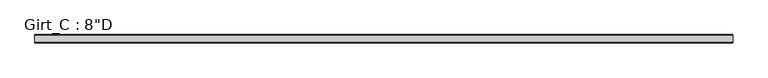
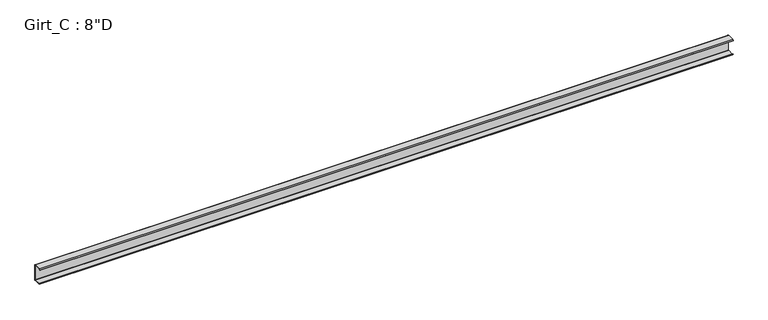
"""IFC4 building model written with IfcOpenShell, lengths in millimetres: beam geometry."""

import ifcopenshell
import ifcopenshell.guid

model = None  # the IFC model being written
_history = None  # IfcOwnerHistory: only IFC2X3 demands one
_inside = {}  # id of a spatial element -> (the spatial element, [elements in it])
_under = {}  # id of a project, library or spatial element -> (it, [spatial elements below it])
_declared = {}  # id of a project -> (the project, [libraries it declares])
_typed = {}  # id of a type object -> (the type object, [elements of that type])
_made_of = {}  # id of a material, layer set ... -> (it, [elements and type objects made of it])


def new_model(schema):
    """Start an empty IFC model of exactly this schema.

    Asked for "IFC4X3", IfcOpenShell would pick the latest addendum, in which some entities
    have other attributes; the version numbers below select the first issue.
    IFC2X3 requires an IfcOwnerHistory on every rooted entity: one is made here for all.
    """
    global model, _history
    if schema == "IFC4X3":
        model = ifcopenshell.file(schema_version=(4, 3, 0, 0))
    else:
        model = ifcopenshell.file(schema=schema)
    _inside.clear()
    _under.clear()
    _declared.clear()
    _typed.clear()
    _made_of.clear()
    _history = None
    if model.schema == "IFC2X3":
        org = make("IfcOrganization", Name="unknown")
        user = make(
            "IfcPersonAndOrganization",
            ThePerson=make("IfcPerson", FamilyName="unknown"),
            TheOrganization=org,
        )
        app = make(
            "IfcApplication",
            ApplicationDeveloper=org,
            Version="unknown",
            ApplicationFullName="unknown",
            ApplicationIdentifier="unknown",
        )
        _history = make(
            "IfcOwnerHistory",
            OwningUser=user,
            OwningApplication=app,
            ChangeAction="ADDED",
            CreationDate=0,
        )
    return model


def make(cls, **values):
    """One entity of the class cls with the attributes given. An attribute that is None is left unset."""
    return model.create_entity(
        cls, **{name: value for name, value in values.items() if value is not None}
    )


def rooted(cls, **values):
    """An entity with a GlobalId (a new one), such as an element, a storey or a relation."""
    return make(cls, GlobalId=ifcopenshell.guid.new(), OwnerHistory=_history, **values)


def si_unit(unit_type, name, prefix=None):
    """IfcSIUnit, for example si_unit("LENGTHUNIT", "METRE", prefix="MILLI")."""
    return make("IfcSIUnit", UnitType=unit_type, Prefix=prefix, Name=name)


def assignment(units):
    """IfcUnitAssignment: the units of a project."""
    return None if units is None else make("IfcUnitAssignment", Units=units)


def point(xyz):
    """IfcCartesianPoint."""
    return None if xyz is None else make("IfcCartesianPoint", Coordinates=xyz)


def direction(xyz):
    """IfcDirection."""
    return None if xyz is None else make("IfcDirection", DirectionRatios=xyz)


def frame(location, z_axis=None, x_axis=None):
    """IfcAxis2Placement3D, a coordinate frame: its origin and axes. An axis left out is left unset."""
    return make(
        "IfcAxis2Placement3D",
        Location=point(location),
        Axis=direction(z_axis),
        RefDirection=direction(x_axis),
    )


def frame_2d(location, x_axis=None):
    """IfcAxis2Placement2D, a coordinate frame in the plane: its origin and x axis."""
    return make(
        "IfcAxis2Placement2D", Location=point(location), RefDirection=direction(x_axis)
    )


def origin():
    """The frame at (0, 0, 0) with its axes left unset."""
    return frame((0.0, 0.0, 0.0))


def place(relative_to, where):
    """IfcLocalPlacement: puts the frame where relative to a parent placement (None: the world)."""
    return make(
        "IfcLocalPlacement", PlacementRelTo=relative_to, RelativePlacement=where
    )


def context(
    kind, dimensions, precision=None, world=None, true_north=None, identifier=None
):
    """IfcGeometricRepresentationContext, for example the 3D "Model" context."""
    return make(
        "IfcGeometricRepresentationContext",
        ContextIdentifier=identifier,
        ContextType=kind,
        CoordinateSpaceDimension=dimensions,
        Precision=precision,
        WorldCoordinateSystem=world,
        TrueNorth=true_north,
    )


def project(units=None, contexts=None):
    """IfcProject with its units and contexts."""
    return rooted(
        "IfcProject",
        Name="project",
        RepresentationContexts=contexts,
        UnitsInContext=assignment(units),
    )


def spatial(cls, under=None, at=None, **own):
    """A site, building, storey or space (cls), placed at a placement, below another one or the project."""
    s = rooted(cls, ObjectPlacement=at, **own)
    if under is not None:
        _under.setdefault(under.id(), (under, []))[1].append(s)
    return s


def polyline(points):
    """IfcPolyline through the points."""
    return make("IfcPolyline", Points=[point(p) for p in points])


def circle_curve(where, radius):
    """IfcCircle in the frame where."""
    return make("IfcCircle", Position=where, Radius=radius)


def trimmed(basis, trim1, trim2, sense, master):
    """IfcTrimmedCurve: the piece of a basis curve between two trims."""
    return make(
        "IfcTrimmedCurve",
        BasisCurve=basis,
        Trim1=trim1,
        Trim2=trim2,
        SenseAgreement=sense,
        MasterRepresentation=master,
    )


def segment(curve, same_sense, transition):
    """IfcCompositeCurveSegment."""
    return make(
        "IfcCompositeCurveSegment",
        Transition=transition,
        SameSense=same_sense,
        ParentCurve=curve,
    )


def composite_curve(segments, self_intersect=None):
    """IfcCompositeCurve: segments joined end to end."""
    return make("IfcCompositeCurve", Segments=segments, SelfIntersect=self_intersect)


def outline(outer, holes=None, kind="AREA"):
    """IfcArbitraryClosedProfileDef: a profile drawn as a closed curve; with holes, ...WithVoids."""
    if holes is None:
        return make("IfcArbitraryClosedProfileDef", ProfileType=kind, OuterCurve=outer)
    return make(
        "IfcArbitraryProfileDefWithVoids",
        ProfileType=kind,
        OuterCurve=outer,
        InnerCurves=holes,
    )


def extrude(swept, where, along, depth):
    """IfcExtrudedAreaSolid: the profile swept, set in the frame where, extruded along a direction by depth."""
    return make(
        "IfcExtrudedAreaSolid",
        SweptArea=swept,
        Position=where,
        ExtrudedDirection=direction(along),
        Depth=depth,
    )


def shape(context_of_items, identifier, shape_type, items):
    """IfcShapeRepresentation: the items that make up one representation, for example the "Body"."""
    return make(
        "IfcShapeRepresentation",
        ContextOfItems=context_of_items,
        RepresentationIdentifier=identifier,
        RepresentationType=shape_type,
        Items=items,
    )


def source(mapping_origin, context_of_items, identifier, shape_type, items):
    """IfcRepresentationMap: a shape defined once, which mapped items show again and again."""
    return make(
        "IfcRepresentationMap",
        MappingOrigin=mapping_origin,
        MappedRepresentation=shape(context_of_items, identifier, shape_type, items),
    )


def transform(
    local_origin,
    x_axis=None,
    y_axis=None,
    z_axis=None,
    scale=None,
    scale2=None,
    scale3=None,
    uniform=True,
):
    """IfcCartesianTransformationOperator3D, or its non-uniform kind. x_axis, y_axis, z_axis: its Axis1, 2, 3."""
    if uniform:
        return make(
            "IfcCartesianTransformationOperator3D",
            Axis1=direction(x_axis),
            Axis2=direction(y_axis),
            LocalOrigin=point(local_origin),
            Scale=scale,
            Axis3=direction(z_axis),
        )
    return make(
        "IfcCartesianTransformationOperator3DnonUniform",
        Axis1=direction(x_axis),
        Axis2=direction(y_axis),
        LocalOrigin=point(local_origin),
        Scale=scale,
        Axis3=direction(z_axis),
        Scale2=scale2,
        Scale3=scale3,
    )


def mapped(mapping_source, mapping_target):
    """IfcMappedItem: shows the shape of a source again, moved by a transform."""
    return make(
        "IfcMappedItem", MappingSource=mapping_source, MappingTarget=mapping_target
    )


def made_of(thing, what):
    """Note that an element or type object is made of a material, layer set ...; save() writes the relation."""
    if what is not None:
        _made_of.setdefault(what.id(), (what, []))[1].append(thing)
    return thing


def element(
    cls,
    number,
    at=None,
    inside=None,
    cuts=None,
    type_object=None,
    material=None,
    context=None,
    identifier="Body",
    shape_type=None,
    held_by="IfcProductDefinitionShape",
    body=None,
    shapes=None,
    **own,
):
    """One element of the class cls, such as IfcWall. Its Tag is "e" and its number.

    at: its placement. inside: the storey or other place that contains it. cuts: it is an
    opening in that element (IfcRelVoidsElement). A single representation is given by context,
    identifier, shape_type and body (its items); several are given by shapes. held_by: the class
    of the entity that holds the representations. save() writes the other relations.
    """
    e = rooted(cls, Tag="e%d" % number, ObjectPlacement=at, **own)
    if body is not None:
        shapes = [shape(context, identifier, shape_type, body)]
    if shapes is not None:
        e.Representation = make(held_by, Representations=shapes)
    if inside is not None:
        _inside.setdefault(inside.id(), (inside, []))[1].append(e)
    if cuts is not None:
        rooted(
            "IfcRelVoidsElement", RelatingBuildingElement=cuts, RelatedOpeningElement=e
        )
    if type_object is not None:
        _typed.setdefault(type_object.id(), (type_object, []))[1].append(e)
    return made_of(e, material)


def aggregate(whole, parts):
    """IfcRelAggregates: a whole, such as a stair, and the parts it consists of."""
    return rooted("IfcRelAggregates", RelatingObject=whole, RelatedObjects=parts)


def save(model, path):
    """Write the relations noted so far, then the file.

    IfcRelAggregates (storeys below a building ...), IfcRelContainedInSpatialStructure (elements
    in a storey), IfcRelDefinesByType, IfcRelAssociatesMaterial and IfcRelDeclares: one each for
    every whole, place, type object, material and project.
    """
    for whole, parts in _under.values():
        aggregate(whole, parts)
    for where, things in _inside.values():
        rooted(
            "IfcRelContainedInSpatialStructure",
            RelatedElements=things,
            RelatingStructure=where,
        )
    for kind, things in _typed.values():
        rooted("IfcRelDefinesByType", RelatedObjects=things, RelatingType=kind)
    for what, things in _made_of.values():
        rooted("IfcRelAssociatesMaterial", RelatedObjects=things, RelatingMaterial=what)
    for by, libraries in _declared.values():
        rooted("IfcRelDeclares", RelatingContext=by, RelatedDefinitions=libraries)
    model.write(path)


def beam_405ad552(model_context):
    return source(origin(), model_context, "Body", "SweptSolid", [
        extrude(outline(composite_curve([segment(polyline([(-87.5109375, 101.6), (-3.3734375, 101.6)]), True, "CONTINUOUS"), segment(trimmed(circle_curve(frame_2d((-3.3734375, 96.8375)), 4.7625), [point((-3.3734375, 101.6))], [point((1.3890625, 96.8375))], False, "CARTESIAN"), True, "CONTINUOUS"), segment(polyline([(1.3890625, 96.8375), (1.3890625, -96.8375)]), True, "CONTINUOUS"), segment(trimmed(circle_curve(frame_2d((-3.3734375, -96.8375)), 4.7625), [point((1.3890625, -96.8375))], [point((-3.3734375, -101.6))], False, "CARTESIAN"), True, "CONTINUOUS"), segment(polyline([(-3.3734375, -101.6), (-87.5109375, -101.6), (-99.7792647, -86.979177), (-97.6510975, -85.1934327), (-86.2154765, -98.821875), (-3.2694106, -98.821875)]), True, "CONTINUOUS"), segment(trimmed(circle_curve(frame_2d((-3.3748024, -96.8389339)), 1.9857399), [point((-3.2694106, -98.821875))], [point((-1.3890625, -96.8389339))], True, "CARTESIAN"), True, "CONTINUOUS"), segment(polyline([(-1.3890625, -96.8389339), (-1.3890625, 96.8381931)]), True, "CONTINUOUS"), segment(trimmed(circle_curve(frame_2d((-3.3741066, 96.8381931)), 1.9850441), [point((-1.3890625, 96.8381931))], [point((-3.3005807, 98.821875))], True, "CARTESIAN"), True, "CONTINUOUS"), segment(polyline([(-3.3005807, 98.821875), (-86.2154765, 98.821875), (-97.6278742, 85.221109), (-99.7560415, 87.0068534), (-87.5109375, 101.6)]), True, "CONTINUOUS")], self_intersect=False)), frame((-4309.3482687, 0.0, 0.0), z_axis=(1.0, 0.0, 0.0), x_axis=(0.0, 1.0, 0.0)), (0.0, 0.0, 1.0), 8560.6732687),
    ])


if __name__ == "__main__":
    model = new_model("IFC4")
    model_context = context("Model", 3, world=origin())
    ifc_project = project(units=[si_unit("LENGTHUNIT", "METRE", prefix="MILLI")], contexts=[model_context])
    site = spatial("IfcSite", under=ifc_project)
    building = spatial("IfcBuilding", under=site)
    placement = place(None, origin())
    beam_shape = beam_405ad552(model_context)
    element("IfcBeam", 1, ObjectType="Girt_C : 8\"D", at=placement, inside=building, context=model_context, shape_type="MappedRepresentation", body=[
        mapped(beam_shape, transform((0.0, 0.0, 0.0), x_axis=(1.0, 0.0, 0.0), y_axis=(0.0, 1.0, 0.0), z_axis=(0.0, 0.0, 1.0))),
    ])
    save(model, "model.ifc")

# Revit data of these elements
# Type "Girt_C : 8\"D"
#   half leg = 0' - 1 3/4"
#   Web_Thickness = 0' - 0 7/64"
#   Length [instance default] = 10' - 0"
#   Leg_1 = 0' - 3 1/2"
#   Height = 0' - 8"
#   Structural Material [instance default] = none
# Element 1 (IfcBeam, "Girt_C : 8\"D")
#   Structural Material = GALVANIZED 'CEE' SECTION (8.0x3.5C - SEE STRUCT. DWGS)
#   Materials on its faces: "GALVANIZED 'CEE' SECTION (8.0x3.5C - SEE STRUCT. DWGS)"
# Materials
#   "GALVANIZED 'CEE' SECTION (8.0x3.5C - SEE STRUCT. DWGS)": class "Metal", colour RGB 137 146 153, transparency 0, Description = "Steel, mill finish", Cost = 0
